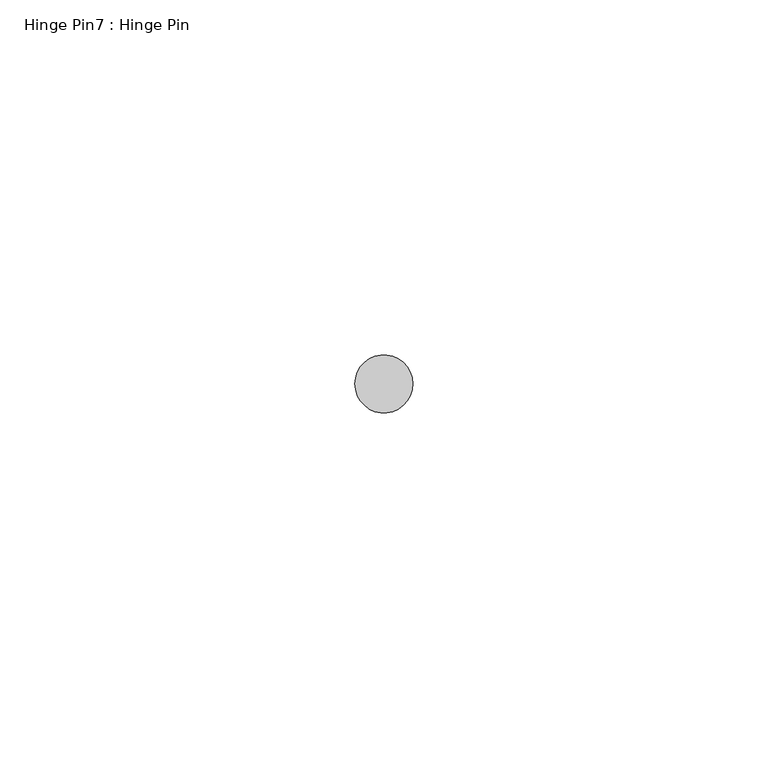
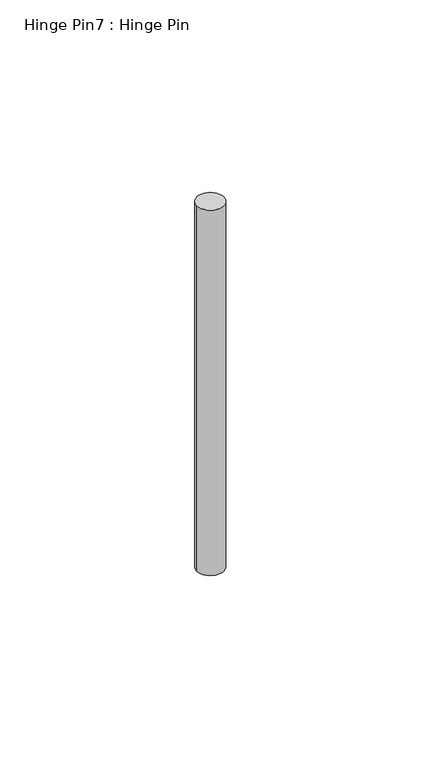
"""IFC4 building model written with IfcOpenShell, lengths in millimetres: proxy geometry, Hinge Pin7 : Hinge Pin."""

from ifc_helpers import new_model, si_unit, point, frame, frame_2d, origin, place, context, project, spatial, circle_curve, trimmed, segment, composite_curve, outline, extrude, source, transform, mapped, element, save


def hinge_pin7_hinge_pin_9f56c2fe(model_context):
    return source(origin(), model_context, "Body", "SweptSolid", [
        extrude(outline(composite_curve([segment(trimmed(circle_curve(frame_2d((587319.1320739, -534100.7049841)), 4.0894), [point((587315.0426739, -534100.7049841))], [point((587323.2214739, -534100.7049841))], False, "CARTESIAN"), True, "CONTINUOUS"), segment(trimmed(circle_curve(frame_2d((587319.1320739, -534100.7049841)), 4.0894), [point((587323.2214739, -534100.7049841))], [point((587315.0426739, -534100.7049841))], False, "CARTESIAN"), True, "CONTINUOUS")], self_intersect=False)), frame((0.0, 0.0, 1941.3140625), z_axis=(0.0, 0.0, 1.0), x_axis=(1.0, 0.0, 0.0)), (0.0, 0.0, 1.0), 117.871875),
    ])


if __name__ == "__main__":
    model = new_model("IFC4")
    model_context = context("Model", 3, world=origin())
    ifc_project = project(units=[si_unit("LENGTHUNIT", "METRE", prefix="MILLI")], contexts=[model_context])
    site = spatial("IfcSite", under=ifc_project)
    building = spatial("IfcBuilding", under=site)
    placement = place(None, origin())
    hinge_pin7_hinge_pin_shape = hinge_pin7_hinge_pin_9f56c2fe(model_context)
    element("IfcBuildingElementProxy", 1, Name="Hinge Pin7 : Hinge Pin", ObjectType="Hinge Pin7 : Hinge Pin", at=placement, inside=building, context=model_context, shape_type="MappedRepresentation", body=[
        mapped(hinge_pin7_hinge_pin_shape, transform((0.0, 0.0, 0.0), x_axis=(1.0, 0.0, 0.0), y_axis=(0.0, 1.0, 0.0), z_axis=(0.0, 0.0, 1.0))),
    ])
    save(model, "model.ifc")

# Revit data of these elements
# Element 1 (IfcBuildingElementProxy, "Hinge Pin7 : Hinge Pin")
#   Materials on its faces: "6\"X6\" WELD-ON STL BUTT HINGE"
# Materials
#   "6\"X6\" WELD-ON STL BUTT HINGE": class "Metal", colour RGB 189 187 185, transparency 0, Description = "Carbon steel", Cost = 0
